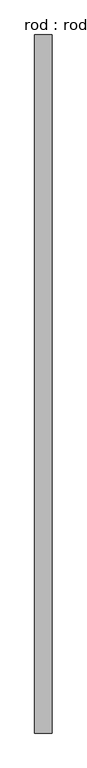
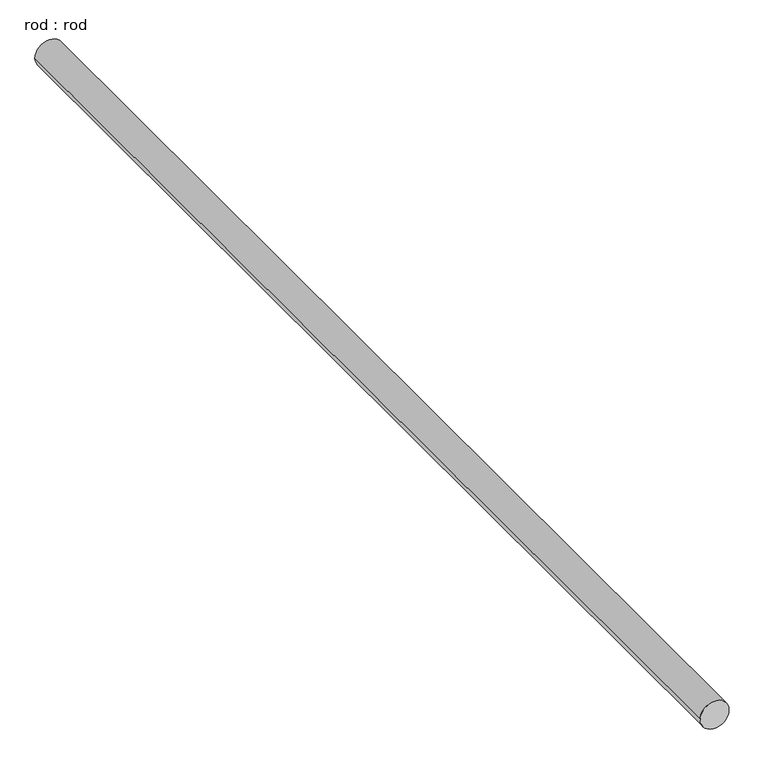
"""IFC4 building model written with IfcOpenShell, lengths in millimetres: proxy geometry, rod : rod."""

from ifc_helpers import new_model, si_unit, point, frame, frame_2d, origin, place, context, project, spatial, circle_curve, trimmed, segment, composite_curve, outline, extrude, source, transform, mapped, element, save


def rod_rod_276faf79(model_context):
    return source(origin(), model_context, "Body", "SweptSolid", [
        extrude(outline(composite_curve([segment(trimmed(circle_curve(frame_2d((0.0108462, 0.0)), 200.0), [point((0.0108462, 200.0))], [point((0.0108462, -200.0))], False, "CARTESIAN"), True, "CONTINUOUS"), segment(trimmed(circle_curve(frame_2d((0.0108462, 0.0)), 200.0), [point((0.0108462, -200.0))], [point((0.0108462, 200.0))], False, "CARTESIAN"), True, "CONTINUOUS")], self_intersect=False)), frame((0.0, -3907.2713847, 0.0), z_axis=(0.0, 1.0, 0.0), x_axis=(0.0, 0.0, 1.0)), (0.0, 0.0, 1.0), 16000.0),
    ])


if __name__ == "__main__":
    model = new_model("IFC4")
    model_context = context("Model", 3, world=origin())
    ifc_project = project(units=[si_unit("LENGTHUNIT", "METRE", prefix="MILLI")], contexts=[model_context])
    site = spatial("IfcSite", under=ifc_project)
    building = spatial("IfcBuilding", under=site)
    placement = place(None, origin())
    rod_rod_shape = rod_rod_276faf79(model_context)
    element("IfcBuildingElementProxy", 1, Name="rod : rod", ObjectType="rod : rod", at=placement, inside=building, context=model_context, shape_type="MappedRepresentation", body=[
        mapped(rod_rod_shape, transform((0.0, 0.0, 0.0), x_axis=(1.0, 0.0, 0.0), y_axis=(0.0, 1.0, 0.0), z_axis=(0.0, 0.0, 1.0))),
    ])
    save(model, "model.ifc")

# Revit data of these elements
# Type "rod : rod"
#   Default Elevation = 0
